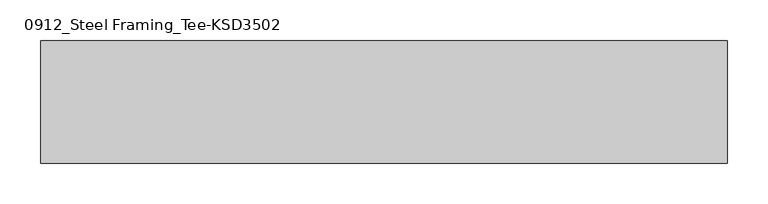
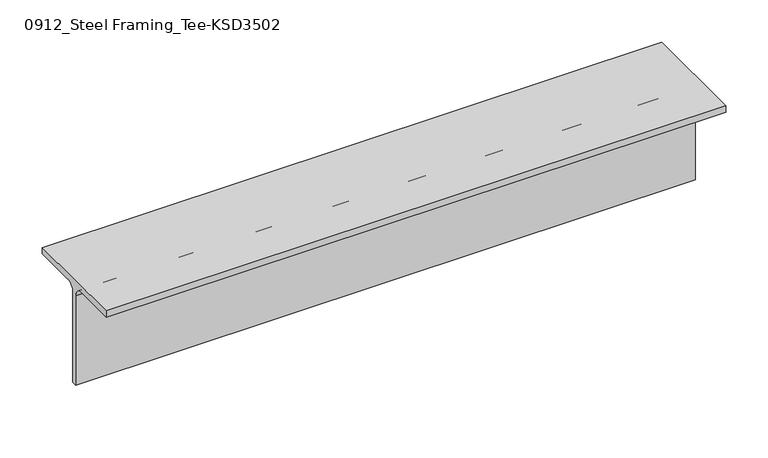
"""IFC4 building model written with IfcOpenShell, lengths in millimetres: member geometry, 0912_Steel Framing_Tee-KSD3502 : H_SB_ASB_CT-150x150x6.5x9."""

from ifc_helpers import new_model, si_unit, point, frame, frame_2d, origin, place, context, project, spatial, polyline, circle_curve, trimmed, segment, composite_curve, outline, extrude, source, transform, mapped, element, save


def member_0912_steel_framing_tee_ksd3502_cf0d02a6(model_context):
    return source(origin(), model_context, "Body", "SweptSolid", [
        extrude(outline(composite_curve([segment(polyline([(-75.0, 75.0), (75.0, 75.0), (75.0, 66.0), (16.25, 66.0)]), True, "CONTINUOUS"), segment(trimmed(circle_curve(frame_2d((16.25, 53.0)), 13.0), [point((16.25, 66.0))], [point((3.25, 53.0))], True, "CARTESIAN"), True, "CONTINUOUS"), segment(polyline([(3.25, 53.0), (3.25, -75.0), (-3.25, -75.0), (-3.25, 53.0)]), True, "CONTINUOUS"), segment(trimmed(circle_curve(frame_2d((-16.25, 53.0)), 13.0), [point((-3.25, 53.0))], [point((-16.25, 66.0))], True, "CARTESIAN"), True, "CONTINUOUS"), segment(polyline([(-16.25, 66.0), (-75.0, 66.0), (-75.0, 75.0)]), True, "CONTINUOUS")], self_intersect=False)), frame((-341.5, 0.0, 0.0), z_axis=(1.0, 0.0, 0.0), x_axis=(0.0, 1.0, 0.0)), (0.0, 0.0, 1.0), 841.5),
    ])


if __name__ == "__main__":
    model = new_model("IFC4")
    model_context = context("Model", 3, world=origin())
    ifc_project = project(units=[si_unit("LENGTHUNIT", "METRE", prefix="MILLI")], contexts=[model_context])
    site = spatial("IfcSite", under=ifc_project)
    building = spatial("IfcBuilding", under=site)
    placement = place(None, origin())
    member_0912_steel_framing_tee_ksd3502_shape = member_0912_steel_framing_tee_ksd3502_cf0d02a6(model_context)
    element("IfcMember", 1, ObjectType="0912_Steel Framing_Tee-KSD3502 : H_SB_ASB_CT-150x150x6.5x9", at=placement, inside=building, context=model_context, shape_type="MappedRepresentation", body=[
        mapped(member_0912_steel_framing_tee_ksd3502_shape, transform((0.0, 0.0, 0.0), x_axis=(1.0, 0.0, 0.0), y_axis=(0.0, 1.0, 0.0), z_axis=(0.0, 0.0, 1.0))),
    ])
    save(model, "model.ifc")

# Revit data of these elements
# Type "0912_Steel Framing_Tee-KSD3502 : H_SB_ASB_CT-150x150x6.5x9"
#   H_WM Code_1 = "S01AA003-00001 | Main Steel Structure Fabrication Work | Shelter/Building | Light Steel - Standard (30KG/M>Weight) | Material: (   )"
#   H_WM Code_2 = "S03AA029-00001 | Main Steel Structure Erection Work | Shelter/Building | Light Steel (30KG/M>Weight) | Material: (   )"
#   H_WM Code_3 = "S01AA010-00001 | Main Steel Structure Fabrication Work | Shelter/Building | Steel Painting/Coating | for Non-Fireproofed Steel Surface, Surface Preparation, Primer, Second & Final Coat | Material: (   )"
#   H_Q'ty Cal Type Tag = "SB-Q2"
#   Width = 15.0 cm
#   Web Thickness = 0.65 cm
#   Web Fillet = 1.3 cm
#   Section Area = 23.39 cm²
#   Perimeter = 0.60 m²/m
#   Nominal Weight = 18.40 kgf/m
#   Height = 15.0 cm
#   Flange Thickness = 0.9 cm
#   Centroid Vertical = 7.5 cm
#   Centroid Horizontal = 7.5 cm
#   Length [instance default] = 1.5000 m
#   Structural Material [instance default] = Steel, 45-345
#   Warping Constant = (empty or 0)
#   Torsional Moment of Inertia = 0
#   Section Name Key = ""
#   Plastic Modulus weak axis = 0
#   Plastic Modulus strong axis = 0
#   Moment of Inertia weak axis = 0
#   Moment of Inertia strong axis = 0
#   Elastic Modulus weak axis = 0
#   Elastic Modulus strong axis = 0
#   Bolt Spacing = 0
#   Assembly Code = ""
# Element 1 (IfcMember, "0912_Steel Framing_Tee-KSD3502 : H_SB_ASB_CT-150x150x6.5x9")
#   Structural Material = none
# Materials
#   "Steel, 45-345": class "Metal", colour RGB 189 187 185, transparency 0, Description = "Steel 345 MPa", Cost = 0
